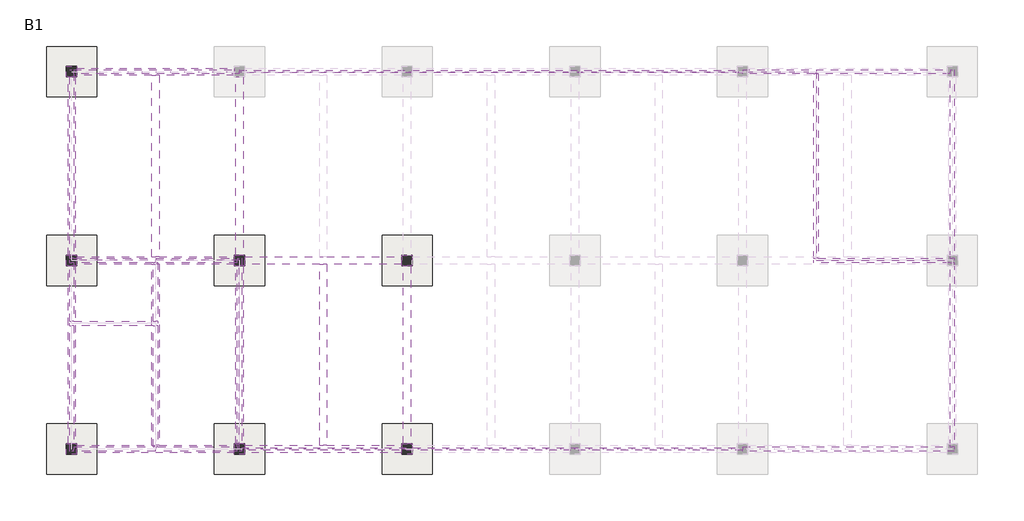
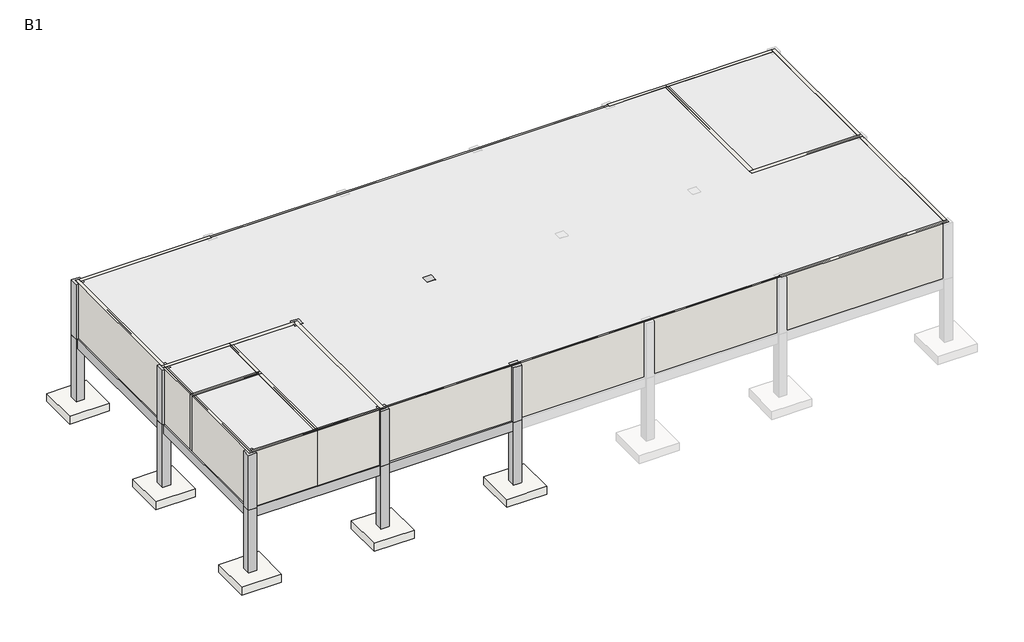
# One storey, part 1 of 2: 21 walls, 14 columns, 13 beams, 12 slabs.
# Revit data of these elements (continued)
# Elements 14, 15, 16, 17, 18, 19, 20, 21, 22, 23, 24, 25, 26, 27 (IfcColumn, "Concrete-Rectangular-Column : CL111_500x500") (continued)
#   Materials on its faces: "콘크리트 - 현장타설 콘크리트"
# Elements 28, 29, 30, 31, 32 (IfcSlab, "CFS11_Slab RC_T150")
#   Height Offset From Level = 0 mm
#   Phase Created = New Construction
#   Materials on its faces: "14200-030101_Concrete Pouring"
# Elements 33, 34, 35, 36, 37, 38, 39 (IfcSlab, "FT112-Footing-Rectangular : FT112_2400x2400x500")
#   Comments = ""
#   hec_material3 = none
#   hec_material2 = none
#   hec_material1 = none
#   Structural Material = 콘크리트 - 현장타설 콘크리트
#   Phase Created = New Construction
#   Materials on its faces: "콘크리트 - 현장타설 콘크리트"
# Elements 40, 42, 45, 46, 47, 49, 50 (IfcWall, "WA111-Exterior RC Wall 200mm")
#   Top Offset = 0 mm
#   Base Offset = 0 mm
#   Unconnected Height = 3500 mm
#   wall height = 3500 mm
#   Phase Created = New Construction
#   Base Constraint = GF
#   Materials on its faces: "Default Wall", "A03AD032-00007_Structural Concrete_25MPa-30MPa"
# Elements 41, 43, 44, 48 (IfcWall, "WA111-Exterior RC Wall 200mm")
#   Top Offset = 0 mm
#   Base Offset = 0 mm
#   Unconnected Height = 3500 mm
#   wall height = 3500 mm
#   Phase Created = New Construction
#   Base Constraint = GF
#   Materials on its faces: "A03AD032-00007_Structural Concrete_25MPa-30MPa", "Default Wall"
# Elements 51, 52 (IfcWall, "WA211_Exterior-Cement Brick-90mm")
#   Top Offset = 0 mm
#   Base Offset = 0 mm
#   Unconnected Height = 3500 mm
#   wall height = 3500 mm
#   Phase Created = New Construction
#   Base Constraint = GF
#   Materials on its faces: "Default Wall", "A04AS164-00002_Plastering_Int", "A04AS164-00001_Plastering_Ext"
# Elements 53, 56, 57, 58 (IfcWall, "WA221_Interior-Cement Block-190mm")
#   Top Offset = 0 mm
#   Base Offset = 0 mm
#   Unconnected Height = 3500 mm
#   wall height = 3500 mm
#   Phase Created = New Construction
#   Base Constraint = GF
#   Materials on its faces: "Default Wall", "A04AS164-00002_Plastering_Int"
# Elements 54, 55, 60 (IfcWall, "WA221_Interior-Cement Block-190mm")
#   Top Offset = 0 mm
#   Base Offset = 0 mm
#   Unconnected Height = 3500 mm
#   wall height = 3500 mm
#   Phase Created = New Construction
#   Base Constraint = GF
#   Materials on its faces: "A04AS164-00002_Plastering_Int", "Default Wall", "A03AD032-00007_Structural Concrete_25MPa-30MPa"
# Element 59 (IfcWall, "WA221_Interior-Cement Block-190mm")
#   Top Offset = 0 mm
#   Base Offset = 0 mm
#   Unconnected Height = 3500 mm
#   wall height = 3500 mm
#   Phase Created = New Construction
#   Base Constraint = GF
#   Materials on its faces: "Default Wall", "A04AS164-00002_Plastering_Int", "A03AD032-00007_Structural Concrete_25MPa-30MPa"
# Materials
#   "콘크리트 - 현장타설 콘크리트": class "콘크리트", colour RGB 192 192 192, transparency 0
#   "A03AE056-00001_Bitumen/Bituminous/Asphalt Coating": class "Generic", colour RGB 17 17 17, transparency 0, Description = "Damp-proofing", W00) Work Master Code = "A03AE056-00001", W01) Work Master_Lv1 = "Concrete Work", W02) Work Master_Lv2 = "Concrete Protective Coating (U/G)", W03) Work Master_Spec.1 = "Bitumen/Bituminous/Asphalt Coating", Cost = 0
#   "A03AC035-00001_Form Work (3 times in use)_Flat": class "Wood", colour RGB 149 120 74, transparency 0, Description = "Plywood", W00) Work Master Code = "A03AC035-00001", W01) Work Master_Lv1 = "Concrete Work", W02) Work Master_Lv2 = "Substructure Work", W03) Work Master_Spec.1 = "Form Work (3 times in use)", W04) Work Master_Spec.2 = "Flat Form", W05) Work Master_Spec.3 = "Dressed Lumber, Plywood or Steel Form(Wood Planks are not Allowed) incl. Chamfer", Cost = 0
#   "A03AC032-00007_Structural Concrete_Type1_25MPa-30Mpa": class "Concrete", colour RGB 176 176 176, transparency 0, Keynote = "09910.A1", Description = "Reinf. Conc.", W00) Work Master Code = "A03AC032-00007", W01) Work Master_Lv1 = "Concrete Work", W02) Work Master_Lv2 = "Substructure Work", W03) Work Master_Spec.1 = "Structural Concrete", W04) Work Master_Spec.2 = "Cement Type-1", W05) Work Master_Spec.3 = "25MPa < F'c (Cylinder Strength) ≤ 30MPa", Cost = 0
#   "14200-030101_Concrete Pouring": class "Concrete", colour RGB 176 176 176, transparency 0, Description = "Reinf. Conc.", W00) Work Master Code = "14200-030101", W01) Work Master_Lv1 = "Concrete Work", W02) Work Master_Lv2 = "Building/Shelter Foundation Work", W03) Work Master_Spec.1 = "Concrete Pouring", W04) Work Master_Spec.2 = "F'c (Cylinder Strength) > 35MPa", W05) Work Master_Spec.3 = "Cement Type-1", Cost = 0
#   "A04AL077-00001_Ext Wall Painting_Acrylic Emulsion Paint": class "Finish", colour RGB 128 128 64, transparency 0, Description = "Plastic", W00) Work Master Code = "A04AL077-00001", W01) Work Master_Lv1 = "Finishing Work", W02) Work Master_Lv2 = "Painting Work", W03) Work Master_Spec.1 = "External Wall Painting", W04) Work Master_Spec.2 = "Acrylic Emulsion Paint", Cost = 0
#   "A03AD032-00007_Structural Concrete_25MPa-30MPa": class "Concrete", colour RGB 176 176 176, transparency 0, Keynote = "09910.A1", Description = "LATEX PAINT ON F.F CONC.", W00) Work Master Code = "A03AD032-00007", W01) Work Master_Lv1 = "Concrete Work", W02) Work Master_Lv2 = "Superstructure Work", W03) Work Master_Spec.1 = "Structural Concrete", W04) Work Master_Spec.2 = "Cement Type-1", W05) Work Master_Spec.3 = "25MPa < F'c (Cylinder Strength) ≤ 30MPa", Cost = 0
#   "A03AD036-00001_Form Work (1 time in use)": class "Wood", colour RGB 149 120 74, transparency 0, Description = "Plywood", W00) Work Master Code = "A03AD036-00001", W01) Work Master_Lv1 = "Concrete Work", W02) Work Master_Lv2 = "Superstructure Work", W03) Work Master_Spec.1 = "Form Work (1 time in use)", W04) Work Master_Spec.2 = "Flat Form", W05) Work Master_Spec.3 = "Dressed Lumber, Plywood or Steel Form(Wood Planks are not Allowed) incl. Chamfer", Cost = 0
#   "A04AL078-00002_Int Wall Painting_Water Emulsion Paint": class "Finish", colour RGB 128 128 64, transparency 0, Description = "Plastic", W00) Work Master Code = "A04AL078-00002", W01) Work Master_Lv1 = "Finishing Work", W02) Work Master_Lv2 = "Painting Work", W03) Work Master_Spec.1 = "Internal Wall Painting", W04) Work Master_Spec.2 = "Water Emulsion Paint", Cost = 0
#   "A04AL081-00001_Skirt_Acrylic Emulsion Paint": class "Finish", colour RGB 128 128 64, transparency 0, Description = "Plastic", W00) Work Master Code = "A04AL081-00001", W01) Work Master_Lv1 = "Finishing Work", W02) Work Master_Lv2 = "Painting Work", W03) Work Master_Spec.1 = "Skirt Painting", W04) Work Master_Spec.2 = "Acrylic Emulsion Paint", W05) Work Master_Spec.3 = "100mm≤H<150mm", Cost = 0
#   "A04AS164-00001_Plastering_Ext": class "Concrete", colour RGB 183 186 184, transparency 0, W00) Work Master Code = "A04AS164-00001", W01) Work Master_Lv1 = "Finishing Work", W02) Work Master_Lv2 = "Plastering Work", W03) Work Master_Spec.1 = "Plastering", W04) Work Master_Spec.2 = "for External Masonry Wall", Cost = 0
#   "A04AK073-00001_Concrete Brick_0.5B": class "Concrete", colour RGB 180 180 180, transparency 0, Description = "Conc. Block", W00) Work Master Code = "A04AK073-00001", W01) Work Master_Lv1 = "Finishing Work", W02) Work Master_Lv2 = "Masonry Work", W03) Work Master_Spec.1 = "Concrete Brick", W04) Work Master_Spec.2 = "[0.5B] w/ All Reinf.(Lath, Steel Tie, Anchor Bar, Mortar, ETC.), Filler, Sealant, Lintel/Sill for Opening, ETC.", Cost = 0
#   "A04AS164-00002_Plastering_Int": class "Concrete", colour RGB 183 186 184, transparency 0, Description = "LATEX PAINT ON THK.15 CEMENT PLASTER", W00) Work Master Code = "A04AS164-00002", W01) Work Master_Lv1 = "Finishing Work", W02) Work Master_Lv2 = "Plastering Work", W03) Work Master_Spec.1 = "Plastering", W04) Work Master_Spec.2 = "for Internal Masonry Wall", Cost = 0
#   "A04AK069-00002_Reinforced Concrete Block_THK 100-200mm": class "Concrete", colour RGB 180 180 180, transparency 0, Description = "Conc. Block", W00) Work Master Code = "A04AK069-00002", W01) Work Master_Lv1 = "Finishing Work", W02) Work Master_Lv2 = "Masonry Work", W03) Work Master_Spec.1 = "Reinforced Concrete Block", W04) Work Master_Spec.2 = "w/ All Reinf.(Lath, Steel Tie, Anchor Bar, Mortar, ETC.), Filler, Sealant, Lintel/Sill for Opening, ETC.", W05) Work Master_Spec.3 = "100mm<THK≤200mm", Cost = 0
#   "Default Wall": class "Miscellaneous", colour RGB 80 80 80, transparency 0
# Room at (84209.652, 177423.861) mm, phase "New Construction", upper offset 3500 mm, lower offset 0 mm
#   Department = "EL"
#   Base Finish = ""
#   Ceiling Finish = "CL2"
#   Wall Finish = "IW2"
#   Floor Finish = "FL7"
#   Number = "0.0"
#   Name = "Battery Room"
#   Interior Finish = "IW2..N/A..N/A,,N/A..N/A,,FL7..N/A,,CL2..N/A"
#   Exterior Finish = "N/A..N/A,,EW2..N/A..N/A"
# Room at (51459.652, 168423.861) mm, phase "New Construction", upper offset 3500 mm, lower offset 0 mm
#   Department = "AR"
#   Base Finish = "WK3"
#   Ceiling Finish = ""
#   Wall Finish = "IW5"
#   Floor Finish = "FL2"
#   Number = "0.1"
#   Name = "Lobby"
#   Interior Finish = "IW5..N/A..N/A,,WK3..N/A,,FL2..N/A,,N/A..N/A"
#   Exterior Finish = "N/A..N/A,,EW2..N/A..N/A"
# Room at (66459.652, 172923.861) mm, phase "New Construction", upper offset 3500 mm, lower offset 0 mm
#   Department = "EL"
#   Base Finish = "WK1"
#   Ceiling Finish = "CL1"
#   Wall Finish = "IW5,IW2"
#   Floor Finish = "FL1"
#   Number = "0.2"
#   Name = "Cable Room"
#   Interior Finish = "IW5..IW2..N/A,,WK1..N/A,,FL1..N/A,,CL1..N/A"
#   Exterior Finish = "N/A..N/A,,EW1..EW2..N/A"
# Room at (47459.652, 166923.861) mm, phase "New Construction", upper offset 3500 mm, lower offset 0 mm
#   Department = "PATHV1"
#   Base Finish = "WK3"
#   Ceiling Finish = "CL1"
#   Wall Finish = "IW5"
#   Floor Finish = "FL2"
#   Number = "0.3"
#   Name = "Stairway"
#   Interior Finish = "IW5..N/A..N/A,,WK3..N/A,,FL2..N/A,,CL1..N/A"
#   Exterior Finish = "N/A..N/A,,EW2..N/A..N/A"
# Room at (47459.652, 171423.861) mm, phase "New Construction", upper offset 3500 mm, lower offset 0 mm
#   Department = "AR"
#   Base Finish = ""
#   Ceiling Finish = "CL3"
#   Wall Finish = ""
#   Floor Finish = ""
#   Number = "0.4"
#   Name = "Elevator"
#   Interior Finish = "N/A..N/A..N/A,,N/A..N/A,,,,CL3..N/A"
#   Exterior Finish = "N/A..N/A,,EW2..N/A..N/A"
